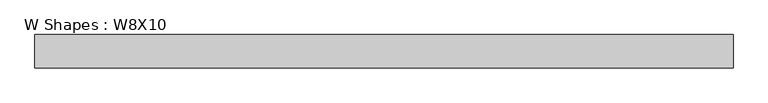
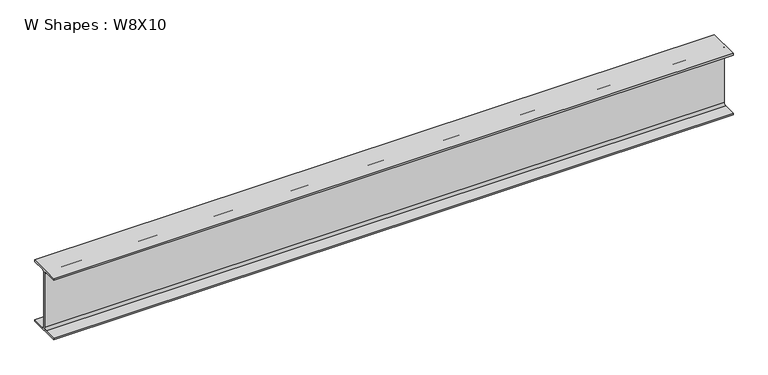
"""IFC4 building model written with IfcOpenShell, lengths in millimetres: beam geometry, W Shapes : W8X10."""

from ifc_helpers import new_model, si_unit, point, frame, frame_2d, origin, place, context, project, spatial, polyline, circle_curve, trimmed, segment, composite_curve, outline, extrude, source, transform, mapped, element, save


def w_shapes_w8x10_5b735649(model_context):
    return source(origin(), model_context, "Body", "SweptSolid", [
        extrude(outline(composite_curve([segment(polyline([(50.038, -94.996), (50.038, -100.203), (-50.038, -100.203), (-50.038, -94.996), (-9.779, -94.996)]), True, "CONTINUOUS"), segment(trimmed(circle_curve(frame_2d((-9.779, -87.376)), 7.62), [point((-9.779, -94.996))], [point((-2.159, -87.376))], True, "CARTESIAN"), True, "CONTINUOUS"), segment(polyline([(-2.159, -87.376), (-2.159, 87.376)]), True, "CONTINUOUS"), segment(trimmed(circle_curve(frame_2d((-9.779, 87.376)), 7.62), [point((-2.159, 87.376))], [point((-9.779, 94.996))], True, "CARTESIAN"), True, "CONTINUOUS"), segment(polyline([(-9.779, 94.996), (-50.038, 94.996), (-50.038, 100.203), (50.038, 100.203), (50.038, 94.996), (9.779, 94.996)]), True, "CONTINUOUS"), segment(trimmed(circle_curve(frame_2d((9.779, 87.376)), 7.62), [point((9.779, 94.996))], [point((2.159, 87.376))], True, "CARTESIAN"), True, "CONTINUOUS"), segment(polyline([(2.159, 87.376), (2.159, -87.376)]), True, "CONTINUOUS"), segment(trimmed(circle_curve(frame_2d((9.779, -87.376)), 7.62), [point((2.159, -87.376))], [point((9.779, -94.996))], True, "CARTESIAN"), True, "CONTINUOUS"), segment(polyline([(9.779, -94.996), (50.038, -94.996)]), True, "CONTINUOUS")], self_intersect=False)), frame((-1049.3744237, 0.0, 0.0), z_axis=(1.0, 0.0, 0.0), x_axis=(0.0, 1.0, 0.0)), (0.0, 0.0, 1.0), 2098.7488474),
    ])


if __name__ == "__main__":
    model = new_model("IFC4")
    model_context = context("Model", 3, world=origin())
    ifc_project = project(units=[si_unit("LENGTHUNIT", "METRE", prefix="MILLI")], contexts=[model_context])
    site = spatial("IfcSite", under=ifc_project)
    building = spatial("IfcBuilding", under=site)
    placement = place(None, origin())
    w_shapes_w8x10_shape = w_shapes_w8x10_5b735649(model_context)
    element("IfcBeam", 1, ObjectType="W Shapes : W8X10", at=placement, inside=building, context=model_context, shape_type="MappedRepresentation", body=[
        mapped(w_shapes_w8x10_shape, transform((0.0, 0.0, 0.0), x_axis=(1.0, 0.0, 0.0), y_axis=(0.0, 1.0, 0.0), z_axis=(0.0, 0.0, 1.0))),
    ])
    save(model, "model.ifc")

# Revit data of these elements
# Type "W Shapes : W8X10"
#   Section Name Key = "W8x10"
#   Assembly Code = "B10"
#   Width = 3.940"
#   Web Thickness = 0.170"
#   Web Fillet = 0.300"
#   Warping Constant = 30.90 in⁶
#   Torsional Moment of Inertia = 0.0426 in⁴
#   Section Area = 2.96 in²
#   Plastic Modulus weak axis = 1.66 in³
#   Plastic Modulus strong axis = 8.87 in³
#   Perimeter = 30.70 ft²/ft
#   Nominal Weight = 10.00 lbf/ft
#   Moment of Inertia weak axis = 2.09 in⁴
#   Moment of Inertia strong axis = 30.80 in⁴
#   Height = 7.890"
#   Flange Thickness = 0.205"
#   Elastic Modulus weak axis = 1.06 in³
#   Elastic Modulus strong axis = 7.81 in³
#   Centroid Vertical = 3.945"
#   Centroid Horizontal = 1.970"
#   Bolt Spacing = 0' - 2 1/4"
#   Length [instance default] = 5' - 0"
#   Structural Material [instance default] = Steel ASTM A992
#   Principal Axes Angle = 0
# Element 1 (IfcBeam, "W Shapes : W8X10")
#   Materials on its faces: "Steel ASTM A992"
# Materials
#   "Steel ASTM A992": class "Metal", colour RGB 199 199 199, transparency 0, Description = "Structural steel 50ksi", Cost = 0
